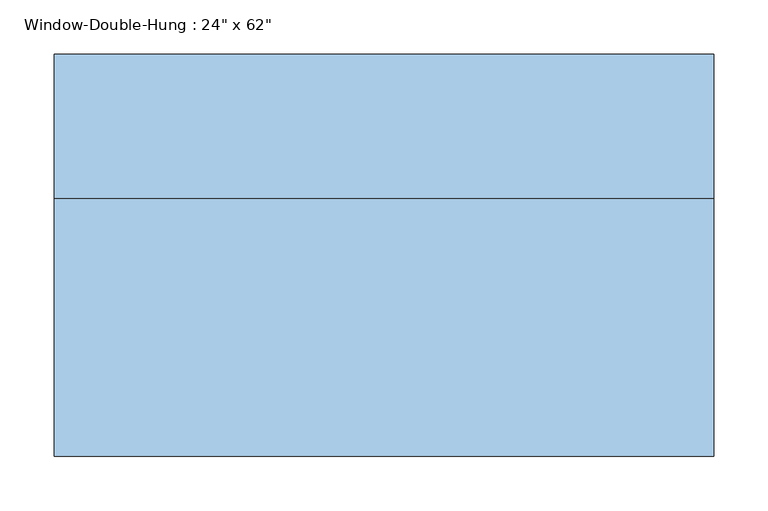
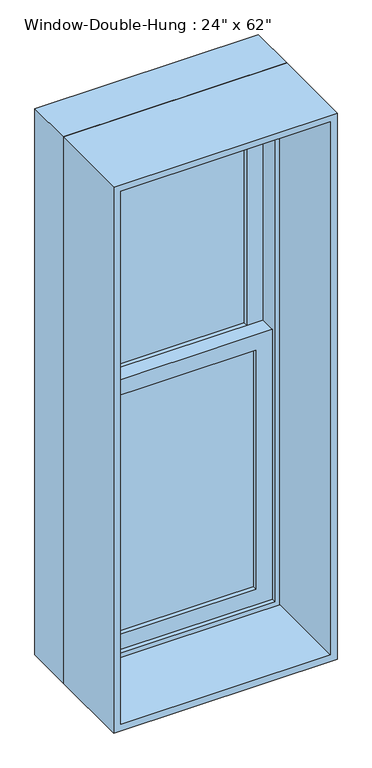
"""IFC4 building model written with IfcOpenShell, lengths in millimetres: window geometry."""

import ifcopenshell
import ifcopenshell.guid

model = None  # the IFC model being written
_history = None  # IfcOwnerHistory: only IFC2X3 demands one
_inside = {}  # id of a spatial element -> (the spatial element, [elements in it])
_under = {}  # id of a project, library or spatial element -> (it, [spatial elements below it])
_declared = {}  # id of a project -> (the project, [libraries it declares])
_typed = {}  # id of a type object -> (the type object, [elements of that type])
_made_of = {}  # id of a material, layer set ... -> (it, [elements and type objects made of it])


def new_model(schema):
    """Start an empty IFC model of exactly this schema.

    Asked for "IFC4X3", IfcOpenShell would pick the latest addendum, in which some entities
    have other attributes; the version numbers below select the first issue.
    IFC2X3 requires an IfcOwnerHistory on every rooted entity: one is made here for all.
    """
    global model, _history
    if schema == "IFC4X3":
        model = ifcopenshell.file(schema_version=(4, 3, 0, 0))
    else:
        model = ifcopenshell.file(schema=schema)
    _inside.clear()
    _under.clear()
    _declared.clear()
    _typed.clear()
    _made_of.clear()
    _history = None
    if model.schema == "IFC2X3":
        org = make("IfcOrganization", Name="unknown")
        user = make(
            "IfcPersonAndOrganization",
            ThePerson=make("IfcPerson", FamilyName="unknown"),
            TheOrganization=org,
        )
        app = make(
            "IfcApplication",
            ApplicationDeveloper=org,
            Version="unknown",
            ApplicationFullName="unknown",
            ApplicationIdentifier="unknown",
        )
        _history = make(
            "IfcOwnerHistory",
            OwningUser=user,
            OwningApplication=app,
            ChangeAction="ADDED",
            CreationDate=0,
        )
    return model


def make(cls, **values):
    """One entity of the class cls with the attributes given. An attribute that is None is left unset."""
    return model.create_entity(
        cls, **{name: value for name, value in values.items() if value is not None}
    )


def rooted(cls, **values):
    """An entity with a GlobalId (a new one), such as an element, a storey or a relation."""
    return make(cls, GlobalId=ifcopenshell.guid.new(), OwnerHistory=_history, **values)


def si_unit(unit_type, name, prefix=None):
    """IfcSIUnit, for example si_unit("LENGTHUNIT", "METRE", prefix="MILLI")."""
    return make("IfcSIUnit", UnitType=unit_type, Prefix=prefix, Name=name)


def assignment(units):
    """IfcUnitAssignment: the units of a project."""
    return None if units is None else make("IfcUnitAssignment", Units=units)


def point(xyz):
    """IfcCartesianPoint."""
    return None if xyz is None else make("IfcCartesianPoint", Coordinates=xyz)


def direction(xyz):
    """IfcDirection."""
    return None if xyz is None else make("IfcDirection", DirectionRatios=xyz)


def frame(location, z_axis=None, x_axis=None):
    """IfcAxis2Placement3D, a coordinate frame: its origin and axes. An axis left out is left unset."""
    return make(
        "IfcAxis2Placement3D",
        Location=point(location),
        Axis=direction(z_axis),
        RefDirection=direction(x_axis),
    )


def origin():
    """The frame at (0, 0, 0) with its axes left unset."""
    return frame((0.0, 0.0, 0.0))


def place(relative_to, where):
    """IfcLocalPlacement: puts the frame where relative to a parent placement (None: the world)."""
    return make(
        "IfcLocalPlacement", PlacementRelTo=relative_to, RelativePlacement=where
    )


def context(
    kind, dimensions, precision=None, world=None, true_north=None, identifier=None
):
    """IfcGeometricRepresentationContext, for example the 3D "Model" context."""
    return make(
        "IfcGeometricRepresentationContext",
        ContextIdentifier=identifier,
        ContextType=kind,
        CoordinateSpaceDimension=dimensions,
        Precision=precision,
        WorldCoordinateSystem=world,
        TrueNorth=true_north,
    )


def project(units=None, contexts=None):
    """IfcProject with its units and contexts."""
    return rooted(
        "IfcProject",
        Name="project",
        RepresentationContexts=contexts,
        UnitsInContext=assignment(units),
    )


def spatial(cls, under=None, at=None, **own):
    """A site, building, storey or space (cls), placed at a placement, below another one or the project."""
    s = rooted(cls, ObjectPlacement=at, **own)
    if under is not None:
        _under.setdefault(under.id(), (under, []))[1].append(s)
    return s


def polyline(points):
    """IfcPolyline through the points."""
    return make("IfcPolyline", Points=[point(p) for p in points])


def outline(outer, holes=None, kind="AREA"):
    """IfcArbitraryClosedProfileDef: a profile drawn as a closed curve; with holes, ...WithVoids."""
    if holes is None:
        return make("IfcArbitraryClosedProfileDef", ProfileType=kind, OuterCurve=outer)
    return make(
        "IfcArbitraryProfileDefWithVoids",
        ProfileType=kind,
        OuterCurve=outer,
        InnerCurves=holes,
    )


def extrude(swept, where, along, depth):
    """IfcExtrudedAreaSolid: the profile swept, set in the frame where, extruded along a direction by depth."""
    return make(
        "IfcExtrudedAreaSolid",
        SweptArea=swept,
        Position=where,
        ExtrudedDirection=direction(along),
        Depth=depth,
    )


def shape(context_of_items, identifier, shape_type, items):
    """IfcShapeRepresentation: the items that make up one representation, for example the "Body"."""
    return make(
        "IfcShapeRepresentation",
        ContextOfItems=context_of_items,
        RepresentationIdentifier=identifier,
        RepresentationType=shape_type,
        Items=items,
    )


def source(mapping_origin, context_of_items, identifier, shape_type, items):
    """IfcRepresentationMap: a shape defined once, which mapped items show again and again."""
    return make(
        "IfcRepresentationMap",
        MappingOrigin=mapping_origin,
        MappedRepresentation=shape(context_of_items, identifier, shape_type, items),
    )


def transform(
    local_origin,
    x_axis=None,
    y_axis=None,
    z_axis=None,
    scale=None,
    scale2=None,
    scale3=None,
    uniform=True,
):
    """IfcCartesianTransformationOperator3D, or its non-uniform kind. x_axis, y_axis, z_axis: its Axis1, 2, 3."""
    if uniform:
        return make(
            "IfcCartesianTransformationOperator3D",
            Axis1=direction(x_axis),
            Axis2=direction(y_axis),
            LocalOrigin=point(local_origin),
            Scale=scale,
            Axis3=direction(z_axis),
        )
    return make(
        "IfcCartesianTransformationOperator3DnonUniform",
        Axis1=direction(x_axis),
        Axis2=direction(y_axis),
        LocalOrigin=point(local_origin),
        Scale=scale,
        Axis3=direction(z_axis),
        Scale2=scale2,
        Scale3=scale3,
    )


def mapped(mapping_source, mapping_target):
    """IfcMappedItem: shows the shape of a source again, moved by a transform."""
    return make(
        "IfcMappedItem", MappingSource=mapping_source, MappingTarget=mapping_target
    )


def made_of(thing, what):
    """Note that an element or type object is made of a material, layer set ...; save() writes the relation."""
    if what is not None:
        _made_of.setdefault(what.id(), (what, []))[1].append(thing)
    return thing


def element(
    cls,
    number,
    at=None,
    inside=None,
    cuts=None,
    type_object=None,
    material=None,
    context=None,
    identifier="Body",
    shape_type=None,
    held_by="IfcProductDefinitionShape",
    body=None,
    shapes=None,
    **own,
):
    """One element of the class cls, such as IfcWall. Its Tag is "e" and its number.

    at: its placement. inside: the storey or other place that contains it. cuts: it is an
    opening in that element (IfcRelVoidsElement). A single representation is given by context,
    identifier, shape_type and body (its items); several are given by shapes. held_by: the class
    of the entity that holds the representations. save() writes the other relations.
    """
    e = rooted(cls, Tag="e%d" % number, ObjectPlacement=at, **own)
    if body is not None:
        shapes = [shape(context, identifier, shape_type, body)]
    if shapes is not None:
        e.Representation = make(held_by, Representations=shapes)
    if inside is not None:
        _inside.setdefault(inside.id(), (inside, []))[1].append(e)
    if cuts is not None:
        rooted(
            "IfcRelVoidsElement", RelatingBuildingElement=cuts, RelatedOpeningElement=e
        )
    if type_object is not None:
        _typed.setdefault(type_object.id(), (type_object, []))[1].append(e)
    return made_of(e, material)


def aggregate(whole, parts):
    """IfcRelAggregates: a whole, such as a stair, and the parts it consists of."""
    return rooted("IfcRelAggregates", RelatingObject=whole, RelatedObjects=parts)


def save(model, path):
    """Write the relations noted so far, then the file.

    IfcRelAggregates (storeys below a building ...), IfcRelContainedInSpatialStructure (elements
    in a storey), IfcRelDefinesByType, IfcRelAssociatesMaterial and IfcRelDeclares: one each for
    every whole, place, type object, material and project.
    """
    for whole, parts in _under.values():
        aggregate(whole, parts)
    for where, things in _inside.values():
        rooted(
            "IfcRelContainedInSpatialStructure",
            RelatedElements=things,
            RelatingStructure=where,
        )
    for kind, things in _typed.values():
        rooted("IfcRelDefinesByType", RelatedObjects=things, RelatingType=kind)
    for what, things in _made_of.values():
        rooted("IfcRelAssociatesMaterial", RelatedObjects=things, RelatingMaterial=what)
    for by, libraries in _declared.values():
        rooted("IfcRelDeclares", RelatingContext=by, RelatedDefinitions=libraries)
    model.write(path)


def window_f919a6bd(model_context):
    return source(origin(), model_context, "Body", "SweptSolid", [
        extrude(outline(polyline([(228.6, 106.3625), (228.6, 100.0125), (-228.6, 100.0125), (-228.6, 106.3625), (228.6, 106.3625)])), frame((0.0, 0.0, 990.6), z_axis=(0.0, 0.0, 1.0), x_axis=(1.0, 0.0, 0.0)), (0.0, 0.0, 1.0), 688.975),
        extrude(outline(polyline([(-228.6, 93.6625), (228.6, 93.6625), (228.6, 87.3125), (-228.6, 87.3125), (-228.6, 93.6625)])), frame((0.0, 0.0, 990.6), z_axis=(0.0, 0.0, 1.0), x_axis=(1.0, 0.0, 0.0)), (0.0, 0.0, 1.0), 688.975),
        extrude(outline(polyline([(228.6, 150.8125), (228.6, 144.4625), (-228.6, 144.4625), (-228.6, 150.8125), (228.6, 150.8125)])), frame((0.0, 0.0, 1724.025), z_axis=(0.0, 0.0, 1.0), x_axis=(1.0, 0.0, 0.0)), (0.0, 0.0, 1.0), 688.975),
        extrude(outline(polyline([(-228.6, 138.1125), (228.6, 138.1125), (228.6, 131.7625), (-228.6, 131.7625), (-228.6, 138.1125)])), frame((0.0, 0.0, 1724.025), z_axis=(0.0, 0.0, 1.0), x_axis=(1.0, 0.0, 0.0)), (0.0, 0.0, 1.0), 688.975),
        extrude(outline(polyline([(1724.025, -273.05), (946.15, -273.05), (946.15, 273.05), (1724.025, 273.05), (1724.025, -273.05)]), holes=[polyline([(1679.575, 228.6), (990.6, 228.6), (990.6, -228.6), (1679.575, -228.6), (1679.575, 228.6)])]), frame((0.0, 74.6125, 0.0), z_axis=(0.0, 1.0, 0.0), x_axis=(0.0, 0.0, 1.0)), (0.0, 0.0, 1.0), 44.45),
        extrude(outline(polyline([(2457.45, -273.05), (1679.575, -273.05), (1679.575, 273.05), (2457.45, 273.05), (2457.45, -273.05)]), holes=[polyline([(2413.0, 228.6), (1724.025, 228.6), (1724.025, -228.6), (2413.0, -228.6), (2413.0, 228.6)])]), frame((0.0, 119.0625, 0.0), z_axis=(0.0, 1.0, 0.0), x_axis=(0.0, 0.0, 1.0)), (0.0, 0.0, 1.0), 44.45),
        extrude(outline(polyline([(2489.2, -304.8), (914.4, -304.8), (914.4, 304.8), (2489.2, 304.8), (2489.2, -304.8)]), holes=[polyline([(2457.45, 273.05), (946.15, 273.05), (946.15, -273.05), (2457.45, -273.05), (2457.45, 273.05)])]), frame((0.0, 61.9125, 0.0), z_axis=(0.0, 1.0, 0.0), x_axis=(0.0, 0.0, 1.0)), (0.0, 0.0, 1.0), 133.35),
        extrude(outline(polyline([(2489.2, 304.8), (2489.2, -304.8), (914.4, -304.8), (914.4, 304.8), (2489.2, 304.8)]), holes=[polyline([(2470.15, 285.75), (933.45, 285.75), (933.45, -285.75), (2470.15, -285.75), (2470.15, 285.75)])]), frame((0.0, -176.2125, 0.0), z_axis=(0.0, 1.0, 0.0), x_axis=(0.0, 0.0, 1.0)), (0.0, 0.0, 1.0), 238.125),
    ])


if __name__ == "__main__":
    model = new_model("IFC4")
    model_context = context("Model", 3, world=origin())
    ifc_project = project(units=[si_unit("LENGTHUNIT", "METRE", prefix="MILLI")], contexts=[model_context])
    site = spatial("IfcSite", under=ifc_project)
    building = spatial("IfcBuilding", under=site)
    placement = place(None, origin())
    window_shape = window_f919a6bd(model_context)
    element("IfcWindow", 1, ObjectType="Window-Double-Hung : 24\" x 62\"", at=placement, inside=building, context=model_context, shape_type="MappedRepresentation", body=[
        mapped(window_shape, transform((0.0, 0.0, 0.0), x_axis=(1.0, 0.0, 0.0), y_axis=(0.0, 1.0, 0.0), z_axis=(0.0, 0.0, 1.0))),
    ])
    save(model, "model.ifc")

# Revit data of these elements
# Type "Window-Double-Hung : 24\" x 62\""
#   Type Mark = "30"
#   Fire Rating = "0.5h"
#   Construction Type Id = "DG-DR"
#   Assembly Code = "B2020100"
#   Analytic Construction = "Double glazing - domestic"
#   Wall Thickness [instance default] = 0' - 6"
#   Window Inset [instance default] = 0' - 0"
#   Visual Light Transmittance = 0.81
#   Thermal Resistance (R) = 1.8146 (h·ft²·°F)/BTU
#   Solar Heat Gain Coefficient = 0.76
#   Muntin Width = 1' - 6"
#   Muntin Height = 2' - 3 1/8"
#   Interior Wall Closure [instance default] = 0' - 1 1/2"
#   Rough Width = 2' - 0 1/2"
#   Rough Height = 5' - 2 1/2"
#   Frame Extension [instance default] = 0' - 1 1/4"
#   Exterior Wall Closure [instance default] = 0' - 0 1/2"
#   Extension Jamb [instance default] = 0' - 1 1/2"
#   Heat Transfer Coefficient (U) = 0.5511 BTU/(h·ft²·°F)
#   Height = 5' - 2"
#   Width = 2' - 0"
#   Top Muntin Visibility = yes
#   Indicator Visibility [instance default] = yes
#   Extension Jamb Visibility [instance default] = yes
#   Interior Trim Visibility [instance default] = yes
#   Exterior Trim Visibility [instance default] = yes
#   Define Thermal Properties by = 1
#   Bottom Muntin Visibility = yes
#   Muntin Pattern = Muntin Pattern_2x2 : Muntin Pattern_2x2
#   Interior Trim Material = Wood - Stained
#   Interior Trim = Trim-Window-Interior-Flat : Picture Frame
#   Exterior Trim Material = Clad - White
#   Exterior Trim = Trim-Window-Exterior-Flat : with Sill
#   Glass Panel Material = Glass
#   Exterior Frame Material = Clad - White
#   Interior Frame Material = Wood - Stained
#   Wall Closure = (empty or 0)
# Element 1 (IfcWindow, "Window-Double-Hung : 24\" x 62\"")
#   Wall Thickness = 1' - 1 7/8"
#   Extension Jamb = 0' - 9 3/8"
#   Materials on its faces: "Wood - Stained", "Glass", "Clad - White"
# Materials
#   "Wood - Stained": class "Wood", colour RGB 224 178 126, transparency 0, Cost = 0
#   "Clad - White": class "Wood", colour RGB 242 242 238, transparency 0, Cost = 0
#   "Glass": class "Glass", colour RGB 0 128 192, transparency 0.75, Description = "Soda Lime Glass", Cost = 0
